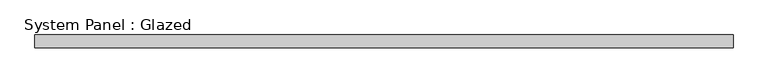
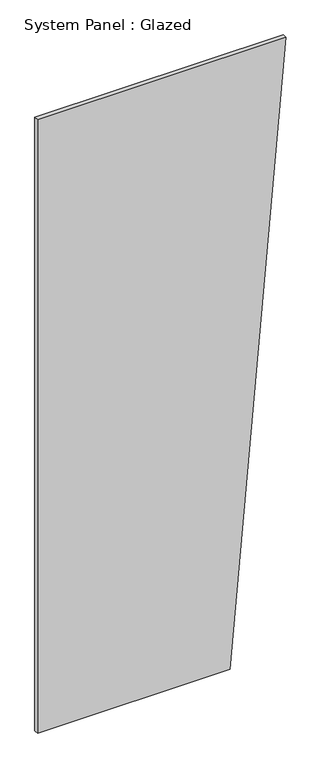
"""IFC4 building model written with IfcOpenShell, lengths in millimetres: plate geometry, System Panel : Glazed."""

import ifcopenshell
import ifcopenshell.guid

model = None  # the IFC model being written
_history = None  # IfcOwnerHistory: only IFC2X3 demands one
_inside = {}  # id of a spatial element -> (the spatial element, [elements in it])
_under = {}  # id of a project, library or spatial element -> (it, [spatial elements below it])
_declared = {}  # id of a project -> (the project, [libraries it declares])
_typed = {}  # id of a type object -> (the type object, [elements of that type])
_made_of = {}  # id of a material, layer set ... -> (it, [elements and type objects made of it])


def new_model(schema):
    """Start an empty IFC model of exactly this schema.

    Asked for "IFC4X3", IfcOpenShell would pick the latest addendum, in which some entities
    have other attributes; the version numbers below select the first issue.
    IFC2X3 requires an IfcOwnerHistory on every rooted entity: one is made here for all.
    """
    global model, _history
    if schema == "IFC4X3":
        model = ifcopenshell.file(schema_version=(4, 3, 0, 0))
    else:
        model = ifcopenshell.file(schema=schema)
    _inside.clear()
    _under.clear()
    _declared.clear()
    _typed.clear()
    _made_of.clear()
    _history = None
    if model.schema == "IFC2X3":
        org = make("IfcOrganization", Name="unknown")
        user = make(
            "IfcPersonAndOrganization",
            ThePerson=make("IfcPerson", FamilyName="unknown"),
            TheOrganization=org,
        )
        app = make(
            "IfcApplication",
            ApplicationDeveloper=org,
            Version="unknown",
            ApplicationFullName="unknown",
            ApplicationIdentifier="unknown",
        )
        _history = make(
            "IfcOwnerHistory",
            OwningUser=user,
            OwningApplication=app,
            ChangeAction="ADDED",
            CreationDate=0,
        )
    return model


def make(cls, **values):
    """One entity of the class cls with the attributes given. An attribute that is None is left unset."""
    return model.create_entity(
        cls, **{name: value for name, value in values.items() if value is not None}
    )


def rooted(cls, **values):
    """An entity with a GlobalId (a new one), such as an element, a storey or a relation."""
    return make(cls, GlobalId=ifcopenshell.guid.new(), OwnerHistory=_history, **values)


def si_unit(unit_type, name, prefix=None):
    """IfcSIUnit, for example si_unit("LENGTHUNIT", "METRE", prefix="MILLI")."""
    return make("IfcSIUnit", UnitType=unit_type, Prefix=prefix, Name=name)


def assignment(units):
    """IfcUnitAssignment: the units of a project."""
    return None if units is None else make("IfcUnitAssignment", Units=units)


def point(xyz):
    """IfcCartesianPoint."""
    return None if xyz is None else make("IfcCartesianPoint", Coordinates=xyz)


def direction(xyz):
    """IfcDirection."""
    return None if xyz is None else make("IfcDirection", DirectionRatios=xyz)


def frame(location, z_axis=None, x_axis=None):
    """IfcAxis2Placement3D, a coordinate frame: its origin and axes. An axis left out is left unset."""
    return make(
        "IfcAxis2Placement3D",
        Location=point(location),
        Axis=direction(z_axis),
        RefDirection=direction(x_axis),
    )


def origin():
    """The frame at (0, 0, 0) with its axes left unset."""
    return frame((0.0, 0.0, 0.0))


def place(relative_to, where):
    """IfcLocalPlacement: puts the frame where relative to a parent placement (None: the world)."""
    return make(
        "IfcLocalPlacement", PlacementRelTo=relative_to, RelativePlacement=where
    )


def context(
    kind, dimensions, precision=None, world=None, true_north=None, identifier=None
):
    """IfcGeometricRepresentationContext, for example the 3D "Model" context."""
    return make(
        "IfcGeometricRepresentationContext",
        ContextIdentifier=identifier,
        ContextType=kind,
        CoordinateSpaceDimension=dimensions,
        Precision=precision,
        WorldCoordinateSystem=world,
        TrueNorth=true_north,
    )


def project(units=None, contexts=None):
    """IfcProject with its units and contexts."""
    return rooted(
        "IfcProject",
        Name="project",
        RepresentationContexts=contexts,
        UnitsInContext=assignment(units),
    )


def spatial(cls, under=None, at=None, **own):
    """A site, building, storey or space (cls), placed at a placement, below another one or the project."""
    s = rooted(cls, ObjectPlacement=at, **own)
    if under is not None:
        _under.setdefault(under.id(), (under, []))[1].append(s)
    return s


def polyline(points):
    """IfcPolyline through the points."""
    return make("IfcPolyline", Points=[point(p) for p in points])


def outline(outer, holes=None, kind="AREA"):
    """IfcArbitraryClosedProfileDef: a profile drawn as a closed curve; with holes, ...WithVoids."""
    if holes is None:
        return make("IfcArbitraryClosedProfileDef", ProfileType=kind, OuterCurve=outer)
    return make(
        "IfcArbitraryProfileDefWithVoids",
        ProfileType=kind,
        OuterCurve=outer,
        InnerCurves=holes,
    )


def extrude(swept, where, along, depth):
    """IfcExtrudedAreaSolid: the profile swept, set in the frame where, extruded along a direction by depth."""
    return make(
        "IfcExtrudedAreaSolid",
        SweptArea=swept,
        Position=where,
        ExtrudedDirection=direction(along),
        Depth=depth,
    )


def shape(context_of_items, identifier, shape_type, items):
    """IfcShapeRepresentation: the items that make up one representation, for example the "Body"."""
    return make(
        "IfcShapeRepresentation",
        ContextOfItems=context_of_items,
        RepresentationIdentifier=identifier,
        RepresentationType=shape_type,
        Items=items,
    )


def source(mapping_origin, context_of_items, identifier, shape_type, items):
    """IfcRepresentationMap: a shape defined once, which mapped items show again and again."""
    return make(
        "IfcRepresentationMap",
        MappingOrigin=mapping_origin,
        MappedRepresentation=shape(context_of_items, identifier, shape_type, items),
    )


def transform(
    local_origin,
    x_axis=None,
    y_axis=None,
    z_axis=None,
    scale=None,
    scale2=None,
    scale3=None,
    uniform=True,
):
    """IfcCartesianTransformationOperator3D, or its non-uniform kind. x_axis, y_axis, z_axis: its Axis1, 2, 3."""
    if uniform:
        return make(
            "IfcCartesianTransformationOperator3D",
            Axis1=direction(x_axis),
            Axis2=direction(y_axis),
            LocalOrigin=point(local_origin),
            Scale=scale,
            Axis3=direction(z_axis),
        )
    return make(
        "IfcCartesianTransformationOperator3DnonUniform",
        Axis1=direction(x_axis),
        Axis2=direction(y_axis),
        LocalOrigin=point(local_origin),
        Scale=scale,
        Axis3=direction(z_axis),
        Scale2=scale2,
        Scale3=scale3,
    )


def mapped(mapping_source, mapping_target):
    """IfcMappedItem: shows the shape of a source again, moved by a transform."""
    return make(
        "IfcMappedItem", MappingSource=mapping_source, MappingTarget=mapping_target
    )


def made_of(thing, what):
    """Note that an element or type object is made of a material, layer set ...; save() writes the relation."""
    if what is not None:
        _made_of.setdefault(what.id(), (what, []))[1].append(thing)
    return thing


def element(
    cls,
    number,
    at=None,
    inside=None,
    cuts=None,
    type_object=None,
    material=None,
    context=None,
    identifier="Body",
    shape_type=None,
    held_by="IfcProductDefinitionShape",
    body=None,
    shapes=None,
    **own,
):
    """One element of the class cls, such as IfcWall. Its Tag is "e" and its number.

    at: its placement. inside: the storey or other place that contains it. cuts: it is an
    opening in that element (IfcRelVoidsElement). A single representation is given by context,
    identifier, shape_type and body (its items); several are given by shapes. held_by: the class
    of the entity that holds the representations. save() writes the other relations.
    """
    e = rooted(cls, Tag="e%d" % number, ObjectPlacement=at, **own)
    if body is not None:
        shapes = [shape(context, identifier, shape_type, body)]
    if shapes is not None:
        e.Representation = make(held_by, Representations=shapes)
    if inside is not None:
        _inside.setdefault(inside.id(), (inside, []))[1].append(e)
    if cuts is not None:
        rooted(
            "IfcRelVoidsElement", RelatingBuildingElement=cuts, RelatedOpeningElement=e
        )
    if type_object is not None:
        _typed.setdefault(type_object.id(), (type_object, []))[1].append(e)
    return made_of(e, material)


def aggregate(whole, parts):
    """IfcRelAggregates: a whole, such as a stair, and the parts it consists of."""
    return rooted("IfcRelAggregates", RelatingObject=whole, RelatedObjects=parts)


def save(model, path):
    """Write the relations noted so far, then the file.

    IfcRelAggregates (storeys below a building ...), IfcRelContainedInSpatialStructure (elements
    in a storey), IfcRelDefinesByType, IfcRelAssociatesMaterial and IfcRelDeclares: one each for
    every whole, place, type object, material and project.
    """
    for whole, parts in _under.values():
        aggregate(whole, parts)
    for where, things in _inside.values():
        rooted(
            "IfcRelContainedInSpatialStructure",
            RelatedElements=things,
            RelatingStructure=where,
        )
    for kind, things in _typed.values():
        rooted("IfcRelDefinesByType", RelatedObjects=things, RelatingType=kind)
    for what, things in _made_of.values():
        rooted("IfcRelAssociatesMaterial", RelatedObjects=things, RelatingMaterial=what)
    for by, libraries in _declared.values():
        rooted("IfcRelDeclares", RelatingContext=by, RelatedDefinitions=libraries)
    model.write(path)


def system_panel_glazed_b3fa7013(model_context):
    return source(origin(), model_context, "Body", "SweptSolid", [
        extrude(outline(polyline([(0.0, -701.3055584), (0.0, 386.1685195), (3657.6, 701.3055584), (3657.6, -701.3055584), (0.0, -701.3055584)])), frame((0.0, -44.45, 0.0), z_axis=(0.0, 1.0, 0.0), x_axis=(0.0, 0.0, 1.0)), (0.0, 0.0, 1.0), 25.4),
    ])


if __name__ == "__main__":
    model = new_model("IFC4")
    model_context = context("Model", 3, world=origin())
    ifc_project = project(units=[si_unit("LENGTHUNIT", "METRE", prefix="MILLI")], contexts=[model_context])
    site = spatial("IfcSite", under=ifc_project)
    building = spatial("IfcBuilding", under=site)
    placement = place(None, origin())
    system_panel_glazed_shape = system_panel_glazed_b3fa7013(model_context)
    element("IfcPlate", 1, ObjectType="System Panel : Glazed", at=placement, inside=building, context=model_context, shape_type="MappedRepresentation", body=[
        mapped(system_panel_glazed_shape, transform((0.0, 0.0, 0.0), x_axis=(1.0, 0.0, 0.0), y_axis=(0.0, 1.0, 0.0), z_axis=(0.0, 0.0, 1.0))),
    ])
    save(model, "model.ifc")

# Revit data of these elements
# Type "System Panel : Glazed"
#   Construction Type Id = "GSP4R"
#   Analytic Construction = "1/8 in Pilkington single glazing"
#   Visual Light Transmittance = 0.9
#   Solar Heat Gain Coefficient = 0.86
#   Heat Transfer Coefficient (U) = 1.18115 BTU/(h·ft²·°F)
#   Define Thermal Properties by = 1
# Element 1 (IfcPlate, "System Panel : Glazed")
#   Materials on its faces: "Glass"
# Materials
#   "Glass": class "Glass", colour RGB 0 128 192, transparency 0.75, Description = "Soda Lime Glass", Cost = 0
